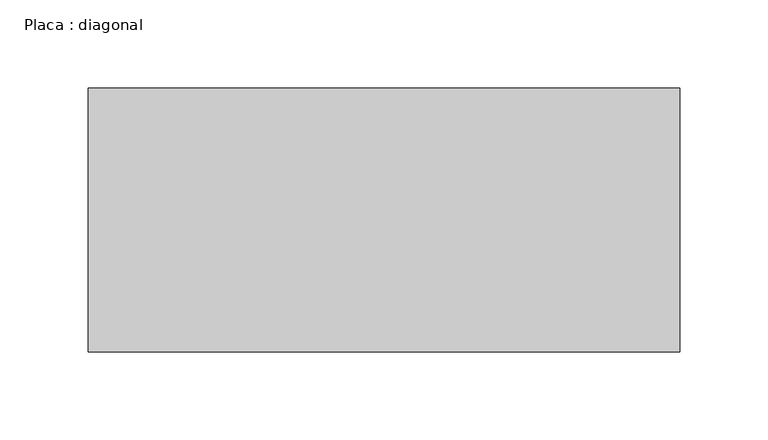
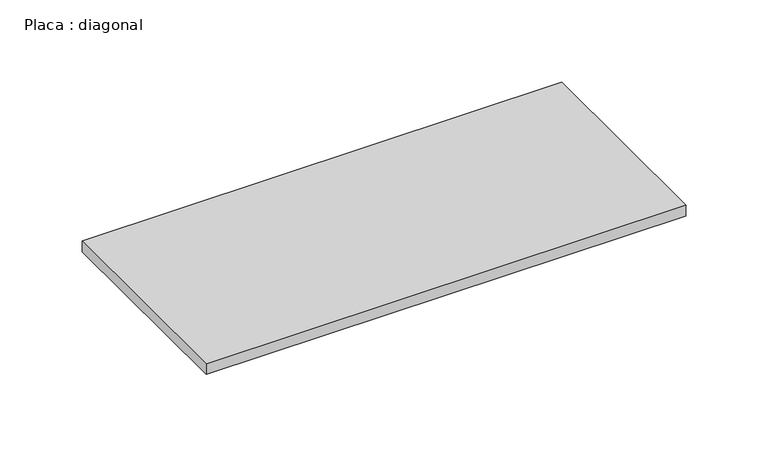
"""IFC4 building model written with IfcOpenShell, lengths in millimetres: beam geometry, Placa : diagonal."""

from ifc_helpers import new_model, si_unit, frame, origin, place, context, project, spatial, polyline, outline, extrude, source, transform, mapped, element, save


def placa_diagonal_fbff302d(model_context):
    return source(origin(), model_context, "Body", "SweptSolid", [
        extrude(outline(polyline([(168.0075515, 75.0), (168.0075515, -75.0), (-168.0075515, -75.0), (-168.0075515, 75.0), (168.0075515, 75.0)])), frame((0.0, 0.0, -4.0), z_axis=(0.0, 0.0, 1.0), x_axis=(1.0, 0.0, 0.0)), (0.0, 0.0, 1.0), 8.0),
    ])


if __name__ == "__main__":
    model = new_model("IFC4")
    model_context = context("Model", 3, world=origin())
    ifc_project = project(units=[si_unit("LENGTHUNIT", "METRE", prefix="MILLI")], contexts=[model_context])
    site = spatial("IfcSite", under=ifc_project)
    building = spatial("IfcBuilding", under=site)
    placement = place(None, origin())
    placa_diagonal_shape = placa_diagonal_fbff302d(model_context)
    element("IfcBeam", 1, ObjectType="Placa : diagonal", at=placement, inside=building, context=model_context, shape_type="MappedRepresentation", body=[
        mapped(placa_diagonal_shape, transform((0.0, 0.0, 0.0), x_axis=(1.0, 0.0, 0.0), y_axis=(0.0, 1.0, 0.0), z_axis=(0.0, 0.0, 1.0))),
    ])
    save(model, "model.ifc")

# Revit data of these elements
# Type "Placa : diagonal"
#   W = 0
#   Length [instance default] = 1.50 m
#   b = 0.15 m
#   d = 0.008 m
#   A = 0 m²
#   Structural Material [instance default] = Aço, 45-345
# Element 1 (IfcBeam, "Placa : diagonal")
#   Materials on its faces: "Aço, 45-345"
# Materials
#   "Aço, 45-345": class "Metal", colour RGB 247 247 247, transparency 0, Description = "Aço 345 MPa", Cost = 0
